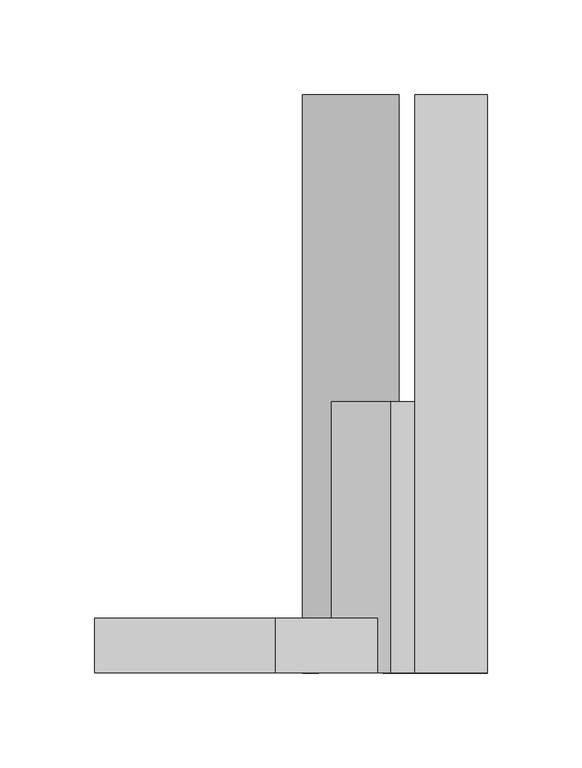
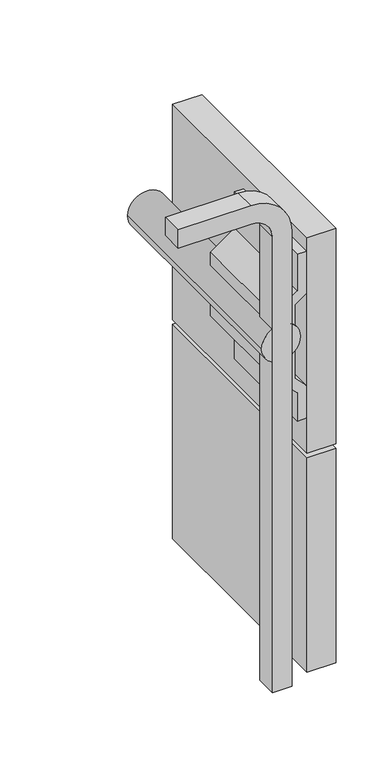
"""IFC4 building model written with IfcOpenShell, lengths in millimetres: proxy geometry, Generic Models 336:Generic Models 334:155419 : Generic Models 336:Generic Models 334:155419."""

from ifc_helpers import new_model, si_unit, point, frame, frame_2d, origin, place, context, project, spatial, polyline, circle_curve, trimmed, segment, composite_curve, outline, extrude, source, transform, mapped, element, save


def generic_models_877177cb(model_context):
    return source(origin(), model_context, "Body", "SweptSolid", [
        extrude(outline(polyline([(8206.5140422, -3919.5173293), (8206.5140422, -3614.7173293), (8244.6140422, -3614.7173293), (8244.6140422, -3919.5173293), (8206.5140422, -3919.5173293)])), frame((0.0, 0.0, 777.875), z_axis=(0.0, 0.0, 1.0), x_axis=(1.0, 0.0, 0.0)), (0.0, 0.0, 1.0), 298.45),
        extrude(outline(polyline([(8206.5140422, -3919.5173293), (8206.5140422, -3614.7173293), (8244.6140422, -3614.7173293), (8244.6140422, -3919.5173293), (8206.5140422, -3919.5173293)])), frame((0.0, 0.0, 474.2011121), z_axis=(0.0, 0.0, 1.0), x_axis=(1.0, 0.0, 0.0)), (0.0, 0.0, 1.0), 297.3238879),
        extrude(outline(composite_curve([segment(polyline([(461.8638344, 8186.6937832), (1092.5918103, 8186.6937832)]), True, "CONTINUOUS"), segment(trimmed(circle_curve(frame_2d((1092.5918103, 8132.8122464)), 53.8815367), [point((1092.5918103, 8186.6937832))], [point((1146.473347, 8132.8122464))], False, "CARTESIAN"), True, "CONTINUOUS"), segment(polyline([(1146.473347, 8132.8122464), (1146.473347, 8037.5622464), (1121.073347, 8037.5622464), (1121.073347, 8132.8122464)]), True, "CONTINUOUS"), segment(trimmed(circle_curve(frame_2d((1092.5918103, 8132.8122464)), 28.4815367), [point((1121.073347, 8132.8122464))], [point((1092.5918103, 8161.2937832))], True, "CARTESIAN"), True, "CONTINUOUS"), segment(polyline([(1092.5918103, 8161.2937832), (461.8638344, 8161.2937832), (461.8638344, 8186.6937832)]), True, "CONTINUOUS")], self_intersect=False)), frame((0.0, -3919.5173293, 0.0), z_axis=(0.0, 1.0, 0.0), x_axis=(0.0, 0.0, 1.0)), (0.0, 0.0, 1.0), 28.9445755),
        extrude(outline(composite_curve([segment(trimmed(circle_curve(frame_2d((942.9201869, 8172.5700497)), 25.4), [point((942.9201869, 8197.9700497))], [point((942.9201869, 8147.1700497))], False, "CARTESIAN"), True, "CONTINUOUS"), segment(trimmed(circle_curve(frame_2d((942.9201869, 8172.5700497)), 25.4), [point((942.9201869, 8147.1700497))], [point((942.9201869, 8197.9700497))], False, "CARTESIAN"), True, "CONTINUOUS")], self_intersect=False)), frame((0.0, -3919.5173293, 0.0), z_axis=(0.0, 1.0, 0.0), x_axis=(0.0, 0.0, 1.0)), (0.0, 0.0, 1.0), 304.8),
        extrude(outline(polyline([(989.2460049, 8190.5511433), (1000.423347, 8206.5140422), (1057.573347, 8206.5140422), (1057.573347, 8193.8140422), (1007.0345486, 8193.8140422), (985.1812864, 8162.6043493), (897.1095726, 8162.6043493), (865.8998797, 8193.8140422), (826.7103919, 8193.8140422), (826.7103919, 8206.5140422), (871.1603919, 8206.5140422), (887.1232908, 8190.5511433), (989.2460049, 8190.5511433)])), frame((0.0, -3919.5173293, 0.0), z_axis=(0.0, 1.0, 0.0), x_axis=(0.0, 0.0, 1.0)), (0.0, 0.0, 1.0), 143.0193921),
    ])


if __name__ == "__main__":
    model = new_model("IFC4")
    model_context = context("Model", 3, world=origin())
    ifc_project = project(units=[si_unit("LENGTHUNIT", "METRE", prefix="MILLI")], contexts=[model_context])
    site = spatial("IfcSite", under=ifc_project)
    building = spatial("IfcBuilding", under=site)
    placement = place(None, origin())
    generic_models_shape = generic_models_877177cb(model_context)
    element("IfcBuildingElementProxy", 1, Name="Generic Models 336:Generic Models 334:155419 : Generic Models 336:Generic Models 334:155419", ObjectType="Generic Models 336:Generic Models 334:155419 : Generic Models 336:Generic Models 334:155419", at=placement, inside=building, context=model_context, shape_type="MappedRepresentation", body=[
        mapped(generic_models_shape, transform((0.0, 0.0, 0.0), x_axis=(1.0, 0.0, 0.0), y_axis=(0.0, 1.0, 0.0), z_axis=(0.0, 0.0, 1.0))),
    ])
    save(model, "model.ifc")

# Revit data of these elements
# Type "Generic Models 336:Generic Models 334:155419 : Generic Models 336:Generic Models 334:155419"
#   NameOverride = "Generic Models 336:Generic Models 334:155419"
#   ObjectTypeOverride = "Generic Models 336:Generic Models 334"
#   Reference = "Generic Models 334"
#   Category = "Generic Models"
#   Tag = "155419"
# Element 1 (IfcBuildingElementProxy, "Generic Models 336:Generic Models 334:155419 : Generic Models 336:Generic Models 334:155419")
#   Materials on its faces: "_GARAGE DOOR TRACK", "_SECTIONAL WOODEN GARAGE DOOR PER SCHEDULE 31400"
# Materials
#   "_GARAGE DOOR TRACK": class "Metal", colour RGB 199 199 199, transparency 0, Description = "Structural steel 50ksi", Cost = 0
#   "_SECTIONAL WOODEN GARAGE DOOR PER SCHEDULE 31400": class "Unassigned", colour RGB 177 130 114, transparency 0
